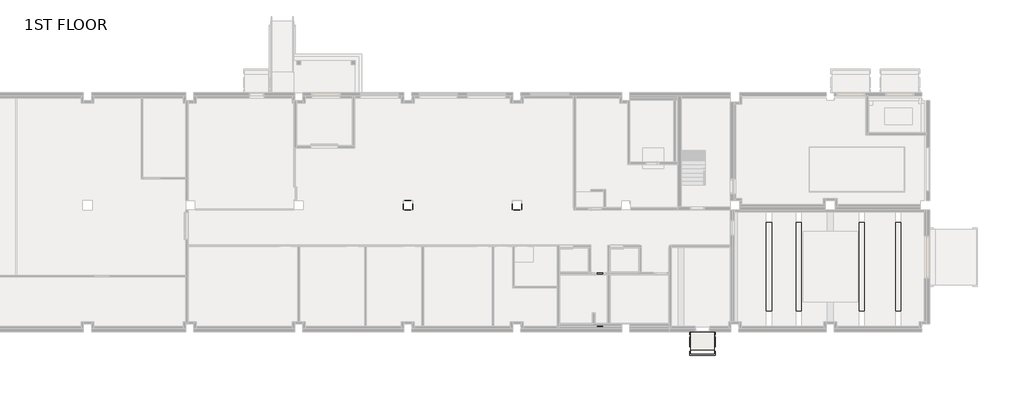
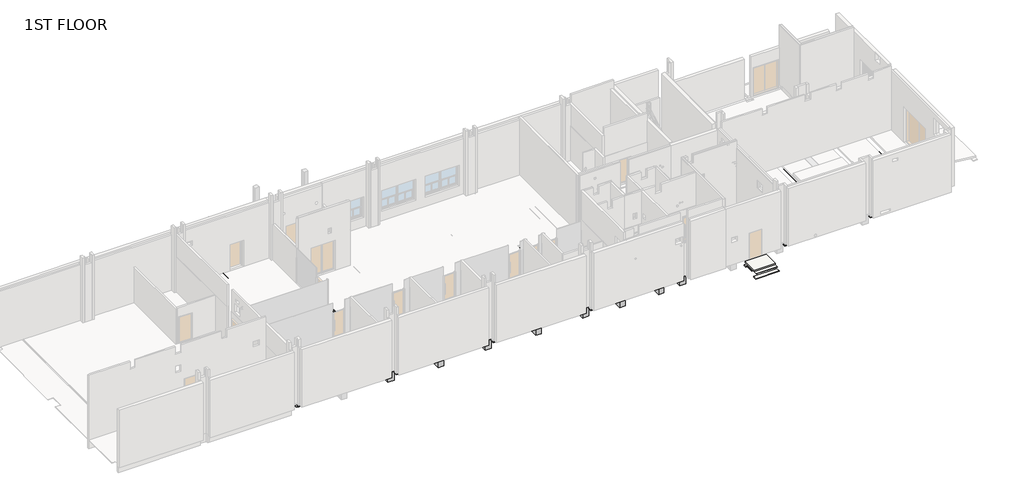
# One storey, part 9 of 15: 19 beams, 7 slabs.
# Revit data of these elements (continued)
# Type "RC Beam_Rectangular : H_SB_AR S16_TG-UG_450x800_1B1B" (continued)
#   중앙부 늑근 = ""
#   외단부 하부근 = ""
#   외단부 상부근 = ""
#   외단부 보조근 = ""
#   외단부 늑근 = ""
#   부호 = "TG3"
#   내단부 하부근 = ""
#   내단부 상부근 = ""
#   내단부 보조근 = ""
#   내단부 늑근 = ""
#   ALL 하부근 = "3-D20"
#   ALL 상부근 = "3-D20"
#   ALL 보조근 = ""
#   ALL 늑근 = "2-D10 @120"
#   H_Rebar Ratio = 0.14
#   Width = 450 mm
#   Height = 800 mm
#   Length [instance default] = 1524 mm
#   b = 450 mm
#   h = 800 mm
#   hec_material3 [instance default] = none
#   hec_material2 [instance default] = none
#   hec_material1 [instance default] = none
#   Structural Material [instance default] = none
#   Assembly Code = ""
# Type "H_SF_AR_B08_Stoop_T150"
#   Type Comments = "CV-AG"
#   H_Rebar Ratio = 0.1
#   Layers, outside or top first: 150 mm "Concrete_f'c=28MPa(Cylender)" (function 1)
# Type "H_SF_AR_B08_Stoop_T125"
#   Type Comments = "CV-AG"
#   H_Rebar Ratio = 0.1
#   Layers, outside or top first: 125 mm "Concrete_f'c=28MPa(Cylender)" (function 1)
# Type "H_SF_AR_S18_Lean_T50"
#   Type Comments = "Lean"
#   Layers, outside or top first: 50 mm "Concrete_f'c=14MPa(Cylender)" (function 1)
# Elements 1, 2, 3, 4 (IfcBeam, "RC Beam_Rectangular : H_SB_AR S16_TG-UG_500x800_1G2")
#   Comments = ""
#   hec_material3 = none
#   hec_material2 = none
#   hec_material1 = none
#   Structural Material = Concrete_f'c=28MPa(Cylender)
#   Phase Created = New Construction
#   Materials on its faces: "Concrete_f'c=28MPa(Cylender)"
# Elements 5, 7, 10, 11, 12 (IfcBeam, "RC Beam_Rectangular : H_SB_AR S16_TG-UG_500x800_1G1")
#   Comments = ""
#   hec_material3 = none
#   hec_material2 = none
#   hec_material1 = none
#   Structural Material = Concrete_f'c=28MPa(Cylender)
#   Phase Created = New Construction
#   Materials on its faces: "Concrete_f'c=28MPa(Cylender)"
# Elements 6, 8, 9 (IfcBeam, "RC Beam_Rectangular : H_SB_AR S16_TG-UG_450x800_1B1")
#   Comments = ""
#   hec_material3 = none
#   hec_material2 = none
#   hec_material1 = none
#   Structural Material = Concrete_f'c=28MPa(Cylender)
#   Phase Created = New Construction
#   Materials on its faces: "Concrete_f'c=28MPa(Cylender)"
# Elements 13, 14, 15 (IfcBeam, "RC Beam_Rectangular : H_SB_AR S16_TG-UG_450x800_1B1A")
#   Comments = ""
#   hec_material3 = none
#   hec_material2 = none
#   hec_material1 = none
#   Structural Material = Concrete_f'c=28MPa(Cylender)
#   Phase Created = New Construction
#   Materials on its faces: "Concrete_f'c=28MPa(Cylender)"
# Element 16 (IfcBeam, "RC Beam_Rectangular : H_SB_AR S16_TG-UG_450x700_1B1B")
#   Comments = ""
#   hec_material3 = none
#   hec_material2 = none
#   hec_material1 = none
#   Structural Material = Concrete_f'c=28MPa(Cylender)
#   Phase Created = New Construction
#   Materials on its faces: "Concrete_f'c=28MPa(Cylender)"
# Element 17 (IfcBeam, "RC Beam_Rectangular : H_SB_AR S16_TG-UG_500x700_1G1A")
#   Comments = ""
#   hec_material3 = none
#   hec_material2 = none
#   hec_material1 = none
#   Structural Material = Concrete_f'c=28MPa(Cylender)
#   Phase Created = New Construction
#   Materials on its faces: "Concrete_f'c=28MPa(Cylender)"
# Element 18 (IfcBeam, "RC Beam_Rectangular : H_SB_AR S16_TG-UG_500x800_1G1A")
#   IfcGUID = "1eK$f4e8T3POk8TBv2woV1"
#   Comments = ""
#   hec_material3 = none
#   hec_material2 = none
#   hec_material1 = none
#   Structural Material = Concrete_f'c=28MPa(Cylender)
#   Phase Created = New Construction
#   Materials on its faces: "Concrete_f'c=28MPa(Cylender)"
# Element 19 (IfcBeam, "RC Beam_Rectangular : H_SB_AR S16_TG-UG_450x800_1B1B")
#   IfcGUID = "1eK$f4e8T3POk8TBv2woGm"
#   Comments = ""
#   hec_material3 = none
#   hec_material2 = none
#   hec_material1 = none
#   Structural Material = Concrete_f'c=28MPa(Cylender)
#   Phase Created = New Construction
#   Materials on its faces: "Concrete_f'c=28MPa(Cylender)"
# Element 20 (IfcSlab, "H_SF_AR_B08_Stoop_T150")
#   Comments = ""
#   built-in parameter 1001955 = -3.14159 (stored number, unit not read)
#   Height Offset From Level = -50 mm
#   built-in parameter 1001954 = 1
#   Phase Created = New Construction
#   Materials on its faces: "Concrete_f'c=28MPa(Cylender)"
# Element 21 (IfcSlab, "H_SF_AR_B08_Stoop_T125")
#   Comments = ""
#   built-in parameter 1001955 = -3.14159 (stored number, unit not read)
#   Height Offset From Level = -175 mm
#   built-in parameter 1001954 = 1
#   Phase Created = New Construction
#   Materials on its faces: "Concrete_f'c=28MPa(Cylender)"
# Element 22 (IfcSlab, "H_SF_AR_S18_Lean_T50")
#   Comments = ""
#   built-in parameter 1001955 = -3.14159 (stored number, unit not read)
#   Height Offset From Level = -500 mm
#   built-in parameter 1001954 = 1
#   Phase Created = New Construction
#   Materials on its faces: "Concrete_f'c=14MPa(Cylender)"
# Element 23 (IfcSlab, "H_SF_AR_S18_Lean_T50")
#   Comments = ""
#   built-in parameter 1001955 = -3.14159 (stored number, unit not read)
#   Height Offset From Level = -350 mm
#   built-in parameter 1001954 = 1
#   Phase Created = New Construction
#   Materials on its faces: "Concrete_f'c=14MPa(Cylender)"
# Element 24 (IfcSlab, "H_SF_AR_S18_Lean_T50")
#   Comments = ""
#   built-in parameter 1001955 = -3.14159 (stored number, unit not read)
#   Height Offset From Level = -200 mm
#   built-in parameter 1001954 = 1
#   Phase Created = New Construction
#   Materials on its faces: "Concrete_f'c=14MPa(Cylender)"
# Element 25 (IfcSlab, "H_SF_AR_S18_Lean_T50")
#   Comments = ""
#   Height Offset From Level = -910 mm
#   built-in parameter 1001954 = 1
#   Phase Created = New Construction
#   Materials on its faces: "Concrete_f'c=14MPa(Cylender)"
# Element 26 (IfcSlab, "H_SF_AR_S18_Lean_T50")
#   Comments = ""
#   Height Offset From Level = -260 mm
#   built-in parameter 1001954 = 1
#   Phase Created = New Construction
#   Materials on its faces: "Concrete_f'c=14MPa(Cylender)"
# Materials
#   "Concrete_f'c=28MPa(Cylender)": class "Concrete", colour RGB 176 176 176, transparency 0, Description = "Reinf. Conc.", Cost = 0, Image = Concrete.Cast-In-Place.Flat.Polished.Grey.jpg
#   "Concrete_f'c=14MPa(Cylender)": class "Concrete", colour RGB 177 177 177, transparency 0, Description = "Reinf. Conc.", Cost = 0
